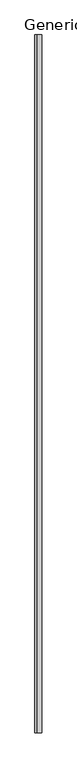
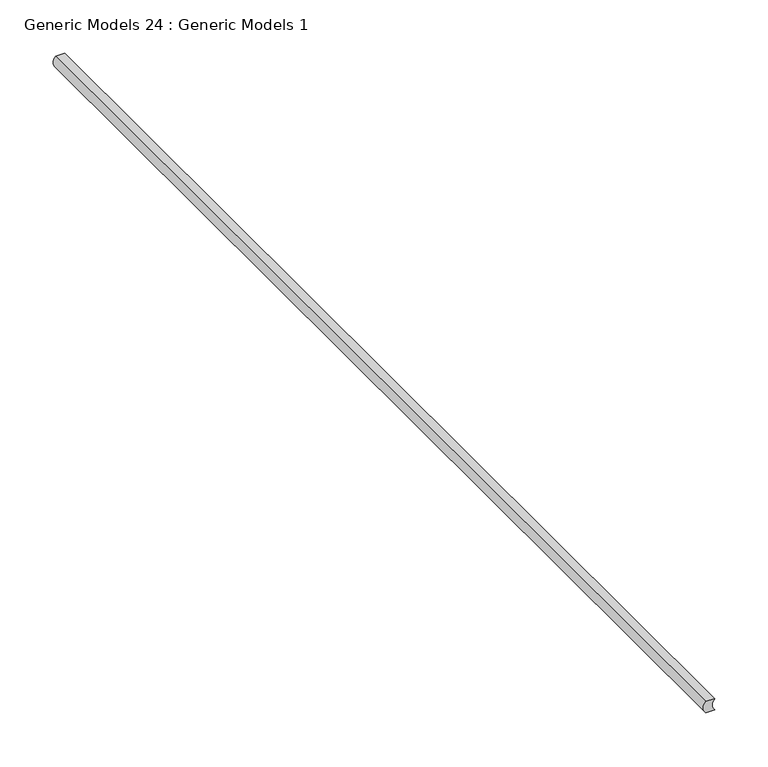
"""IFC4 building model written with IfcOpenShell, lengths in millimetres: proxy geometry, Generic Models 24 : Generic Models 1."""

from ifc_helpers import new_model, si_unit, point, frame, frame_2d, origin, place, context, project, spatial, polyline, circle_curve, trimmed, segment, composite_curve, outline, extrude, source, transform, mapped, element, save


def generic_models_24_generic_models_1_5dd0a967(model_context):
    return source(origin(), model_context, "Body", "SweptSolid", [
        extrude(outline(composite_curve([segment(trimmed(circle_curve(frame_2d((526.6526794, 52672.1490918)), 8.620055), [point((520.3026794, 52666.3196108))], [point((533.0026794, 52666.3196108))], True, "CARTESIAN"), True, "CONTINUOUS"), segment(polyline([(533.0026794, 52666.3196108), (533.0026794, 52656.7946108)]), True, "CONTINUOUS"), segment(trimmed(circle_curve(frame_2d((526.6526794, 52662.6240918)), 8.620055), [point((533.0026794, 52656.7946108))], [point((520.3026794, 52656.7946108))], False, "CARTESIAN"), True, "CONTINUOUS"), segment(polyline([(520.3026794, 52656.7946108), (520.3026794, 52666.3196108)]), True, "CONTINUOUS")], self_intersect=False)), frame((0.0, 0.0, 0.0), z_axis=(0.0, 1.0, 0.0), x_axis=(0.0, 0.0, 1.0)), (0.0, 0.0, 1.0), 1219.2),
    ])


if __name__ == "__main__":
    model = new_model("IFC4")
    model_context = context("Model", 3, world=origin())
    ifc_project = project(units=[si_unit("LENGTHUNIT", "METRE", prefix="MILLI")], contexts=[model_context])
    site = spatial("IfcSite", under=ifc_project)
    building = spatial("IfcBuilding", under=site)
    placement = place(None, origin())
    generic_models_24_generic_models_1_shape = generic_models_24_generic_models_1_5dd0a967(model_context)
    element("IfcBuildingElementProxy", 1, Name="Generic Models 24 : Generic Models 1", ObjectType="Generic Models 24 : Generic Models 1", at=placement, inside=building, context=model_context, shape_type="MappedRepresentation", body=[
        mapped(generic_models_24_generic_models_1_shape, transform((0.0, 0.0, 0.0), x_axis=(1.0, 0.0, 0.0), y_axis=(0.0, 1.0, 0.0), z_axis=(0.0, 0.0, 1.0))),
    ])
    save(model, "model.ifc")

# Revit data of these elements
# Element 1 (IfcBuildingElementProxy, "Generic Models 24 : Generic Models 1")
#   Materials on its faces: "ACOUSTICAL SEALANT"
# Materials
#   "ACOUSTICAL SEALANT": class "Unassigned", colour RGB 120 120 120, transparency 0, Cost = 0
